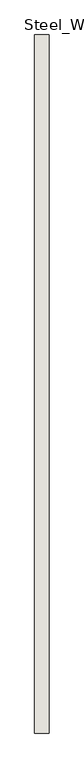
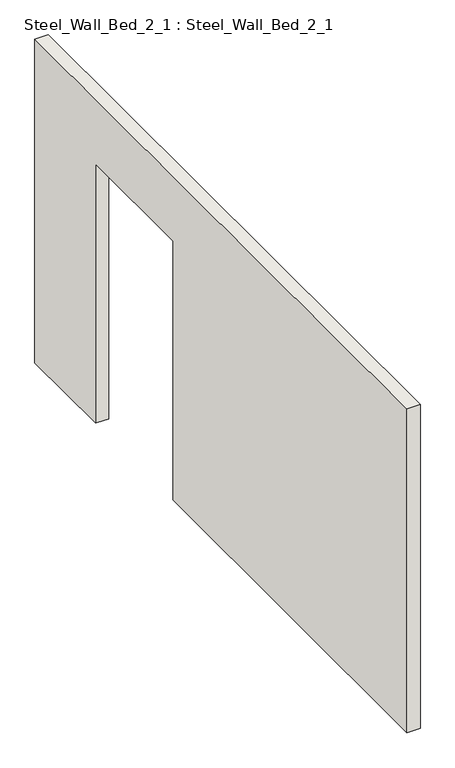
"""IFC4 building model written with IfcOpenShell, lengths in millimetres: wall geometry, Steel_Wall_Bed_2_1 : Steel_Wall_Bed_2_1."""

from ifc_helpers import new_model, si_unit, frame, origin, place, context, project, spatial, polyline, outline, extrude, source, transform, mapped, element, save


def steel_wall_bed_2_1_steel_wall_bed_2_1_f0eb02fb(model_context):
    return source(origin(), model_context, "Body", "SweptSolid", [
        extrude(outline(polyline([(4695.0, 2850.0), (9595.0, 2850.0), (9595.0, 250.0), (8795.0, 250.0), (8795.0, 2330.0), (7775.0, 2330.0), (7775.0, 250.0), (4695.0, 250.0), (4695.0, 2850.0)])), frame((1515.0, 0.0, 0.0), z_axis=(1.0, 0.0, 0.0), x_axis=(0.0, 1.0, 0.0)), (0.0, 0.0, 1.0), 100.0),
    ])


if __name__ == "__main__":
    model = new_model("IFC4")
    model_context = context("Model", 3, world=origin())
    ifc_project = project(units=[si_unit("LENGTHUNIT", "METRE", prefix="MILLI")], contexts=[model_context])
    site = spatial("IfcSite", under=ifc_project)
    building = spatial("IfcBuilding", under=site)
    placement = place(None, origin())
    steel_wall_bed_2_1_steel_wall_bed_2_1_shape = steel_wall_bed_2_1_steel_wall_bed_2_1_f0eb02fb(model_context)
    element("IfcWall", 1, ObjectType="Steel_Wall_Bed_2_1 : Steel_Wall_Bed_2_1", at=placement, inside=building, context=model_context, shape_type="MappedRepresentation", body=[
        mapped(steel_wall_bed_2_1_steel_wall_bed_2_1_shape, transform((0.0, 0.0, 0.0), x_axis=(1.0, 0.0, 0.0), y_axis=(0.0, 1.0, 0.0), z_axis=(0.0, 0.0, 1.0))),
    ])
    save(model, "model.ifc")

# Revit data of these elements
# Type "Steel_Wall_Bed_2_1 : Steel_Wall_Bed_2_1"
#   NameOverride = "Steel_Wall_Bed_2_1"
# Element 1 (IfcWall, "Steel_Wall_Bed_2_1 : Steel_Wall_Bed_2_1")
#   Materials on its faces: "IfcSurfaceStyle #33"
# Materials
#   "IfcSurfaceStyle #33": class "Unassigned", colour RGB 214 214 214, transparency 0
